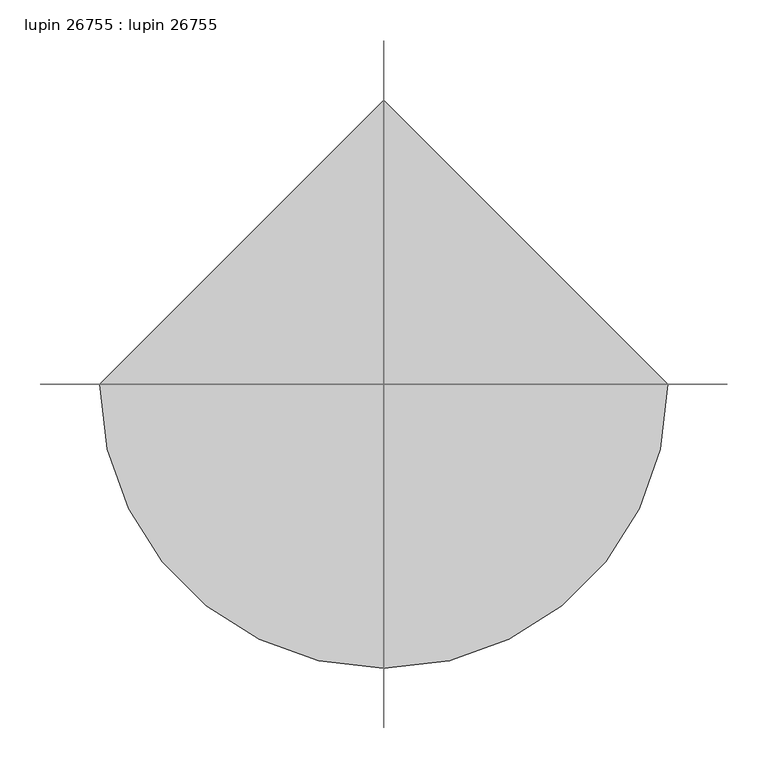
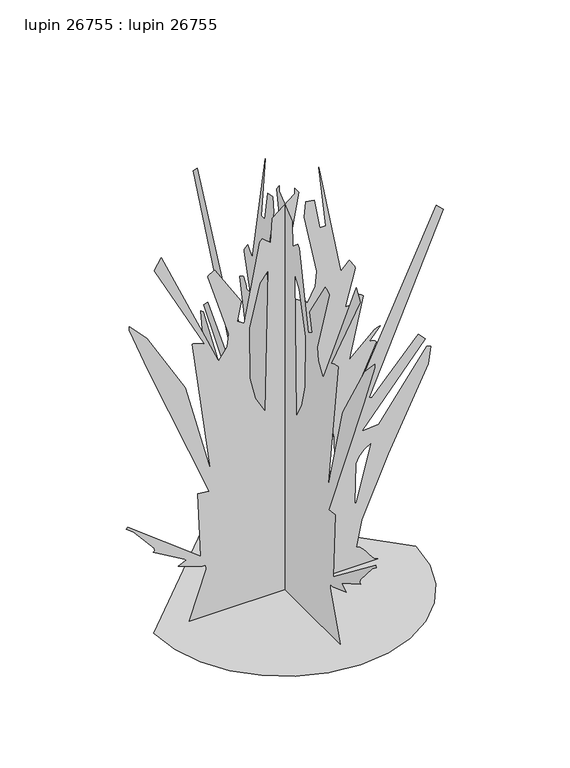
"""IFC4 building model written with IfcOpenShell, lengths in millimetres: proxy geometry, lupin 26755 : lupin 26755."""

import ifcopenshell
import ifcopenshell.guid

model = None  # the IFC model being written
_history = None  # IfcOwnerHistory: only IFC2X3 demands one
_inside = {}  # id of a spatial element -> (the spatial element, [elements in it])
_under = {}  # id of a project, library or spatial element -> (it, [spatial elements below it])
_declared = {}  # id of a project -> (the project, [libraries it declares])
_typed = {}  # id of a type object -> (the type object, [elements of that type])
_made_of = {}  # id of a material, layer set ... -> (it, [elements and type objects made of it])


def new_model(schema):
    """Start an empty IFC model of exactly this schema.

    Asked for "IFC4X3", IfcOpenShell would pick the latest addendum, in which some entities
    have other attributes; the version numbers below select the first issue.
    IFC2X3 requires an IfcOwnerHistory on every rooted entity: one is made here for all.
    """
    global model, _history
    if schema == "IFC4X3":
        model = ifcopenshell.file(schema_version=(4, 3, 0, 0))
    else:
        model = ifcopenshell.file(schema=schema)
    _inside.clear()
    _under.clear()
    _declared.clear()
    _typed.clear()
    _made_of.clear()
    _history = None
    if model.schema == "IFC2X3":
        org = make("IfcOrganization", Name="unknown")
        user = make(
            "IfcPersonAndOrganization",
            ThePerson=make("IfcPerson", FamilyName="unknown"),
            TheOrganization=org,
        )
        app = make(
            "IfcApplication",
            ApplicationDeveloper=org,
            Version="unknown",
            ApplicationFullName="unknown",
            ApplicationIdentifier="unknown",
        )
        _history = make(
            "IfcOwnerHistory",
            OwningUser=user,
            OwningApplication=app,
            ChangeAction="ADDED",
            CreationDate=0,
        )
    return model


def make(cls, **values):
    """One entity of the class cls with the attributes given. An attribute that is None is left unset."""
    return model.create_entity(
        cls, **{name: value for name, value in values.items() if value is not None}
    )


def rooted(cls, **values):
    """An entity with a GlobalId (a new one), such as an element, a storey or a relation."""
    return make(cls, GlobalId=ifcopenshell.guid.new(), OwnerHistory=_history, **values)


def si_unit(unit_type, name, prefix=None):
    """IfcSIUnit, for example si_unit("LENGTHUNIT", "METRE", prefix="MILLI")."""
    return make("IfcSIUnit", UnitType=unit_type, Prefix=prefix, Name=name)


def assignment(units):
    """IfcUnitAssignment: the units of a project."""
    return None if units is None else make("IfcUnitAssignment", Units=units)


def point(xyz):
    """IfcCartesianPoint."""
    return None if xyz is None else make("IfcCartesianPoint", Coordinates=xyz)


def direction(xyz):
    """IfcDirection."""
    return None if xyz is None else make("IfcDirection", DirectionRatios=xyz)


def frame(location, z_axis=None, x_axis=None):
    """IfcAxis2Placement3D, a coordinate frame: its origin and axes. An axis left out is left unset."""
    return make(
        "IfcAxis2Placement3D",
        Location=point(location),
        Axis=direction(z_axis),
        RefDirection=direction(x_axis),
    )


def origin():
    """The frame at (0, 0, 0) with its axes left unset."""
    return frame((0.0, 0.0, 0.0))


def place(relative_to, where):
    """IfcLocalPlacement: puts the frame where relative to a parent placement (None: the world)."""
    return make(
        "IfcLocalPlacement", PlacementRelTo=relative_to, RelativePlacement=where
    )


def context(
    kind, dimensions, precision=None, world=None, true_north=None, identifier=None
):
    """IfcGeometricRepresentationContext, for example the 3D "Model" context."""
    return make(
        "IfcGeometricRepresentationContext",
        ContextIdentifier=identifier,
        ContextType=kind,
        CoordinateSpaceDimension=dimensions,
        Precision=precision,
        WorldCoordinateSystem=world,
        TrueNorth=true_north,
    )


def project(units=None, contexts=None):
    """IfcProject with its units and contexts."""
    return rooted(
        "IfcProject",
        Name="project",
        RepresentationContexts=contexts,
        UnitsInContext=assignment(units),
    )


def spatial(cls, under=None, at=None, **own):
    """A site, building, storey or space (cls), placed at a placement, below another one or the project."""
    s = rooted(cls, ObjectPlacement=at, **own)
    if under is not None:
        _under.setdefault(under.id(), (under, []))[1].append(s)
    return s


def point_list(points):
    """IfcCartesianPointList2D or 3D."""
    cls = (
        "IfcCartesianPointList2D" if len(points[0]) == 2 else "IfcCartesianPointList3D"
    )
    return make(cls, CoordList=points)


def triangles(points, corners, closed=None, point_numbers=None):
    """IfcTriangulatedFaceSet: each triangle names its three corners, points numbered from 1."""
    return make(
        "IfcTriangulatedFaceSet",
        Coordinates=point_list(points),
        Closed=closed,
        CoordIndex=corners,
        PnIndex=point_numbers,
    )


def shape(context_of_items, identifier, shape_type, items):
    """IfcShapeRepresentation: the items that make up one representation, for example the "Body"."""
    return make(
        "IfcShapeRepresentation",
        ContextOfItems=context_of_items,
        RepresentationIdentifier=identifier,
        RepresentationType=shape_type,
        Items=items,
    )


def source(mapping_origin, context_of_items, identifier, shape_type, items):
    """IfcRepresentationMap: a shape defined once, which mapped items show again and again."""
    return make(
        "IfcRepresentationMap",
        MappingOrigin=mapping_origin,
        MappedRepresentation=shape(context_of_items, identifier, shape_type, items),
    )


def transform(
    local_origin,
    x_axis=None,
    y_axis=None,
    z_axis=None,
    scale=None,
    scale2=None,
    scale3=None,
    uniform=True,
):
    """IfcCartesianTransformationOperator3D, or its non-uniform kind. x_axis, y_axis, z_axis: its Axis1, 2, 3."""
    if uniform:
        return make(
            "IfcCartesianTransformationOperator3D",
            Axis1=direction(x_axis),
            Axis2=direction(y_axis),
            LocalOrigin=point(local_origin),
            Scale=scale,
            Axis3=direction(z_axis),
        )
    return make(
        "IfcCartesianTransformationOperator3DnonUniform",
        Axis1=direction(x_axis),
        Axis2=direction(y_axis),
        LocalOrigin=point(local_origin),
        Scale=scale,
        Axis3=direction(z_axis),
        Scale2=scale2,
        Scale3=scale3,
    )


def mapped(mapping_source, mapping_target):
    """IfcMappedItem: shows the shape of a source again, moved by a transform."""
    return make(
        "IfcMappedItem", MappingSource=mapping_source, MappingTarget=mapping_target
    )


def made_of(thing, what):
    """Note that an element or type object is made of a material, layer set ...; save() writes the relation."""
    if what is not None:
        _made_of.setdefault(what.id(), (what, []))[1].append(thing)
    return thing


def element(
    cls,
    number,
    at=None,
    inside=None,
    cuts=None,
    type_object=None,
    material=None,
    context=None,
    identifier="Body",
    shape_type=None,
    held_by="IfcProductDefinitionShape",
    body=None,
    shapes=None,
    **own,
):
    """One element of the class cls, such as IfcWall. Its Tag is "e" and its number.

    at: its placement. inside: the storey or other place that contains it. cuts: it is an
    opening in that element (IfcRelVoidsElement). A single representation is given by context,
    identifier, shape_type and body (its items); several are given by shapes. held_by: the class
    of the entity that holds the representations. save() writes the other relations.
    """
    e = rooted(cls, Tag="e%d" % number, ObjectPlacement=at, **own)
    if body is not None:
        shapes = [shape(context, identifier, shape_type, body)]
    if shapes is not None:
        e.Representation = make(held_by, Representations=shapes)
    if inside is not None:
        _inside.setdefault(inside.id(), (inside, []))[1].append(e)
    if cuts is not None:
        rooted(
            "IfcRelVoidsElement", RelatingBuildingElement=cuts, RelatedOpeningElement=e
        )
    if type_object is not None:
        _typed.setdefault(type_object.id(), (type_object, []))[1].append(e)
    return made_of(e, material)


def aggregate(whole, parts):
    """IfcRelAggregates: a whole, such as a stair, and the parts it consists of."""
    return rooted("IfcRelAggregates", RelatingObject=whole, RelatedObjects=parts)


def save(model, path):
    """Write the relations noted so far, then the file.

    IfcRelAggregates (storeys below a building ...), IfcRelContainedInSpatialStructure (elements
    in a storey), IfcRelDefinesByType, IfcRelAssociatesMaterial and IfcRelDeclares: one each for
    every whole, place, type object, material and project.
    """
    for whole, parts in _under.values():
        aggregate(whole, parts)
    for where, things in _inside.values():
        rooted(
            "IfcRelContainedInSpatialStructure",
            RelatedElements=things,
            RelatingStructure=where,
        )
    for kind, things in _typed.values():
        rooted("IfcRelDefinesByType", RelatedObjects=things, RelatingType=kind)
    for what, things in _made_of.values():
        rooted("IfcRelAssociatesMaterial", RelatedObjects=things, RelatingMaterial=what)
    for by, libraries in _declared.values():
        rooted("IfcRelDeclares", RelatingContext=by, RelatedDefinitions=libraries)
    model.write(path)


def lupin_26755_lupin_26755_1db73bb0(model_context):
    return source(origin(), model_context, "Body", "Tessellation", [
        triangles([(-351.9469769, 0.0, 0.0), (-342.6429663, -80.6431063, 0.0), (-316.1457464, -154.7010223, 0.0), (-274.573611, -220.0515756, 0.0), (-220.0515756, -274.573611, 0.0), (-154.700768, -316.1457464, 0.0), (-80.6431063, -342.6429663, 0.0), (1.54e-05, -351.9469769, 0.0), (80.6431063, -342.6429663, 0.0), (154.7010223, -316.1457464, 0.0), (220.0515756, -274.573611, 0.0), (274.573611, -220.0515756, 0.0), (316.1457464, -154.700768, 0.0), (342.6429663, -80.6431063, 0.0), (351.9469769, 3.08e-05, 0.0), (-4.62e-05, 351.9469769, 0.0), (150.6720804, -0.0015947, 851.9910187), (173.2724542, -0.0015961, 874.5918921), (188.3394669, -0.0015947, 851.9910187), (188.5203062, -0.0015944, 847.0684994), (161.9722718, -0.0015884, 746.5202036), (177.0392664, -0.0015884, 746.5202036), (178.9694175, -0.0015886, 750.284436), (180.6039107, -0.0015889, 754.0461977), (182.1639718, -0.0015891, 757.8054159), (183.8723704, -0.0015893, 761.5671049), (185.9508409, -0.0015895, 765.3339535), (188.6214083, -0.0015898, 769.1058163), (192.1062791, -0.00159, 772.8878529), (193.2812801, -0.00159, 772.4611347), (195.5106317, -0.0015899, 771.3080074), (198.4649026, -0.0015898, 769.6264967), (201.8143893, -0.0015897, 767.6173897), (205.2296787, -0.0015896, 765.4761686), (208.3815575, -0.0015894, 763.4010046), (210.9401041, -0.0015893, 761.5874525), (173.2724542, -0.0015792, 592.0833366), (240.700733, -0.0015829, 654.2395718), (250.6943454, -0.0015832, 659.6218014), (256.1408516, -0.0015833, 659.8859568), (226.0070987, -0.0015812, 625.984683), (228.5658996, -0.0015812, 626.1598904), (231.7175241, -0.0015812, 625.7001801), (235.1327953, -0.0015812, 624.7324339), (238.4825545, -0.0015811, 623.3938528), (241.4365711, -0.001581, 621.8114639), (243.6659227, -0.0015809, 620.1197794), (244.8409236, -0.0015808, 618.4509859), (180.8060786, -0.0015725, 479.0814042), (184.572909, -0.0015725, 479.0814042), (406.8108882, -0.0016005, 949.9256659), (425.6449857, -0.0015994, 931.0915684), (226.0070987, -0.0015718, 467.7809675), (233.5407231, -0.0015716, 464.0141553), (357.8448363, -0.0015797, 599.6169611), (376.6763904, -0.0015785, 580.7828636), (207.1732737, -0.0015664, 377.3799811), (252.3745481, -0.0015666, 381.1467934), (380.4432026, -0.0015772, 558.1819902), (391.7436393, -0.001577, 554.4177215), (384.6443633, -0.0015741, 506.8385036), (278.1600926, -0.0015612, 289.3386073), (206.7572381, -0.0015515, 126.6752076), (192.1062791, -0.0015471, 53.437713), (201.6487926, -0.0015469, 49.4892894), (210.1163717, -0.0015464, 41.8553304), (217.9390592, -0.0015458, 32.010051), (225.5471159, -0.0015452, 21.427562), (233.3697852, -0.0015446, 11.5823576), (241.8373824, -0.0015442, 3.9483989), (251.3798959, -0.0015439, 1.66e-05), (-256.5091613, -0.001544, 0.4898205), (-211.4973739, -0.0015518, 132.0554297), (-212.2487088, -0.0015525, 144.4635658), (-222.2372343, -0.0015525, 143.8397394), (-286.2728424, -0.0015538, 166.4403676), (-263.6719508, -0.0015545, 177.7405681), (-354.0729735, -0.0015577, 230.4752126), (-348.9472326, -0.0015578, 232.5839138), (-351.022433, -0.0015583, 241.0403199), (-406.3257797, -0.0015621, 305.3939318), (-425.6424422, -0.0015631, 320.8777614), (-421.87563, -0.0015633, 324.6445736), (-226.0037922, -0.0015543, 173.9740102), (-233.5374348, -0.0015651, 354.7790714), (-203.4034275, -0.0015648, 351.0122592), (-366.5443417, -0.0015886, 750.3606668), (-417.7760619, -0.0015966, 882.9891266), (-418.1088178, -0.0015972, 893.4259169), (-370.8775801, -0.0015942, 843.3371864), (-268.1575782, -0.0015837, 667.2316566), (-199.6365971, -0.0015682, 407.5119355), (-248.6044294, -0.0015907, 784.1883259), (-246.3971695, -0.0015907, 784.2213181), (-242.3227634, -0.0015906, 783.3755121), (-236.9745433, -0.0015905, 781.8490065), (-230.9453692, -0.0015904, 779.8398268), (-224.8285369, -0.0015903, 777.5436733), (-219.2169245, -0.0015901, 775.1611879), (-214.7036098, -0.00159, 772.8878529), (-350.306125, -0.0016053, 1029.028759), (-331.4720638, -0.0016071, 1059.1632568), (-180.8027903, -0.0015866, 716.3881765), (-177.0359781, -0.0015864, 712.6214006), (-155.1577168, -0.0015883, 744.8692142), (-150.1099781, -0.0015904, 779.1769312), (-207.1702397, -0.0016012, 961.2260662), (-205.9949844, -0.0016013, 963.0370749), (-203.7656147, -0.0016014, 965.1147823), (-194.0468402, -0.0016018, 970.9440777), (-190.8949614, -0.0016019, 972.0972776), (-188.3364148, -0.0016019, 972.5265392), (-116.7679544, -0.0015952, 859.5246431), (-128.0681458, -0.001592, 806.7891993), (-109.2343208, -0.0015913, 795.4887989), (-67.8001221, -0.0016041, 1010.1946615), (-60.2664931, -0.0016046, 1017.728286), (-37.6658604, -0.0016035, 998.8941885), (-33.8993003, -0.0016075, 1066.6968813), (26.3689732, -0.0016104, 1115.6629332), (26.3689732, -0.0016113, 1130.7301821), (37.6691624, -0.0016104, 1115.6629332), (2.9836067, -0.0015988, 921.19319), (5.2254839, -0.0015953, 862.2830503), (21.4607608, -0.0015927, 818.4376162), (56.5029828, -0.0015916, 799.2555748), (60.269795, -0.0015911, 791.7219503), (81.2288264, -0.0015936, 833.4109028), (86.0914021, -0.0015961, 874.8052511), (51.7460784, -0.0016059, 1039.955781), (56.5029828, -0.0016084, 1081.7615868), (79.10362, -0.0016082, 1077.9948109), (94.1706237, -0.0016032, 995.1274126), (109.237373, -0.0016032, 995.1274126), (90.4038023, -0.0016136, 1168.3983044), (-67.325905, -0.0015972, 893.4183592), (-96.1172708, -0.0015902, 776.6851501), (-94.9783414, -0.0015817, 633.9373953), (-79.6923831, -0.001578, 571.2782112), (-52.7331184, -0.0015752, 524.2831873), (-45.1994894, -0.001599, 923.5579439), (109.237373, -0.0015608, 283.2096027), (135.6048224, -0.0015619, 302.0436639), (131.8382554, -0.0015682, 407.5119355), (211.912919, -0.0015632, 322.7039944), (198.2078507, -0.0015623, 307.9059877), (189.9752137, -0.0015612, 290.5146256), (188.3394669, -0.0015547, 181.5073803), (192.1062791, -0.0015545, 177.7405681), (232.2618404, -0.0015639, 335.5792259), (0.0016106, 150.6687739, 851.9910187), (0.0016109, 173.269402, 874.5918921), (0.00161, 188.3364148, 851.9910187), (0.0016099, 188.5169997, 847.0684994), (0.0016073, 161.9689653, 746.5202036), (0.001607, 177.0362324, 746.5202036), (0.0016071, 178.9663653, 750.284436), (0.0016072, 180.6006042, 754.0461977), (0.0016073, 182.1609196, 757.8054159), (0.0016074, 183.8693182, 761.5671049), (0.0016075, 185.9478069, 765.3339535), (0.0016076, 188.6183561, 769.1058163), (0.0016076, 192.103227, 772.8878529), (0.0016076, 193.2782279, 772.4611347), (0.0016075, 195.5075795, 771.3080074), (0.0016074, 198.4615962, 769.6264967), (0.0016073, 201.8113554, 767.6173897), (0.0016072, 205.2266265, 765.4761686), (0.0016071, 208.378251, 763.4010046), (0.001607, 210.937052, 761.5874525), (0.0016025, 173.269402, 592.0833366), (0.0016033, 240.6974266, 654.2395718), (0.0016034, 250.6910389, 659.6218014), (0.0016033, 256.1383082, 659.8859568), (0.0016027, 226.0040465, 625.984683), (0.0016027, 228.5625931, 626.1598904), (0.0016026, 231.7142176, 625.7001801), (0.0016026, 235.1297431, 624.7324339), (0.0016025, 238.479248, 623.3938528), (0.0016024, 241.4332646, 621.8114639), (0.0016023, 243.6626162, 620.1197794), (0.0016022, 244.8378715, 618.4509859), (0.001599, 180.8027903, 479.0814042), (0.001599, 184.5696025, 479.0814042), (0.0016097, 406.8083447, 949.9256659), (0.0016088, 425.6424422, 931.0915684), (0.001598, 226.0040465, 467.7809675), (0.0015978, 233.5374348, 464.0141553), (0.0016, 357.8397858, 599.6169611), (0.0015991, 376.6738469, 580.7828636), (0.0015956, 207.1702397, 377.3799811), (0.001595, 252.3712416, 381.1467934), (0.0015984, 380.4406591, 558.1845337), (0.0015981, 391.7410958, 554.4177215), (0.0015968, 384.6418199, 506.8385036), (0.0015919, 278.1575492, 289.3386073), (0.0015881, 206.7539316, 126.6752076), (0.0015862, 192.103227, 53.437713), (0.0015859, 201.6454861, 49.4892894), (0.0015856, 210.1130652, 41.8553304), (0.0015851, 217.936007, 32.010051), (0.0015847, 225.5438094, 21.427587), (0.0015843, 233.3664787, 11.5823837), (0.001584, 241.8343303, 3.9483989), (0.0015837, 251.3765894, 2.41e-05), (0.0015913, -256.51423, 0.4898434), (0.0015945, -211.5006804, 132.0554297), (0.0015949, -212.2519971, 144.4635658), (0.001595, -222.2402864, 143.8397394), (0.0015967, -286.2753676, 166.4403676), (0.0015967, -263.6744943, 177.7405681), (0.0015996, -354.0780241, 230.4752126), (0.0015996, -348.9497761, 232.5839138), (0.0015999, -351.0249764, 241.0403199), (0.0016026, -406.3308303, 305.3939318), (0.0016033, -425.6449857, 320.8777614), (0.0016034, -421.8781734, 324.6445736), (0.001596, -226.0070987, 173.9740102), (0.0016015, -233.5404688, 354.7790714), (0.0016009, -203.4064615, 351.0122592), (0.0016153, -366.5468851, 750.3606668), (0.00162, -417.7786054, 882.9891266), (0.0016203, -418.1113612, 893.4259169), (0.0016181, -370.8801235, 843.3371864), (0.0016113, -268.1626651, 667.2316566), (0.0016026, -199.6396492, 407.5119355), (0.0016145, -248.6077359, 784.1883259), (0.0016145, -246.4002216, 784.2213181), (0.0016144, -242.3260699, 783.3755121), (0.0016143, -236.9775955, 781.8490065), (0.0016141, -230.9484032, 779.8398268), (0.001614, -224.8318434, 777.5436733), (0.0016138, -219.2199766, 775.1611879), (0.0016137, -214.7069163, 772.8878529), (0.0016233, -350.3112119, 1029.028759), (0.0016239, -331.4771507, 1059.1632568), (0.0016115, -180.8060786, 716.3881765), (0.0016113, -177.0392664, 712.6214006), (0.001612, -155.1607508, 744.8692142), (0.0016129, -150.1132755, 779.1769312), (0.0016192, -207.1732737, 961.2260662), (0.0016192, -205.9982728, 963.0396183), (0.0016192, -203.7689212, 965.1147823), (0.0016193, -194.0498742, 970.9466211), (0.0016193, -190.8979953, 972.0998211), (0.0016192, -188.3394669, 972.5265392), (0.0016148, -116.7709974, 859.5246431), (0.0016134, -128.0714432, 806.7891993), (0.0016128, -109.2376273, 795.4887989), (0.0016186, -67.8031697, 1010.1946615), (0.0016187, -60.269795, 1017.728286), (0.0016178, -37.6691624, 998.8941885), (0.0016197, -33.9023479, 1066.6968813), (0.0016203, 26.3656713, 1115.6629332), (0.0016207, 26.3656713, 1130.7301821), (0.0016201, 37.6661148, 1115.6629332), (0.0016148, 2.9804319, 921.19319), (0.0016131, 5.2223085, 862.2830503), (0.0016115, 21.4575588, 818.4376162), (0.0016104, 56.4999352, 799.2555748), (0.0016101, 60.2664931, 791.7219503), (0.0016111, 81.225529, 833.4109028), (0.0016122, 86.0883499, 874.8052511), (0.0016177, 51.7430263, 1039.955781), (0.0016188, 56.4999352, 1081.7615868), (0.0016184, 79.1003135, 1077.9948109), (0.0016157, 94.1673172, 995.1274126), (0.0016155, 109.2340665, 995.1274126), (0.0016209, 90.4007593, 1168.3983044), (0.0016151, -67.329207, 893.4183592), (0.001612, -96.120323, 776.6851501), (0.0016077, -94.9816388, 633.9373953), (0.0016057, -79.6956896, 571.2782112), (0.0016039, -52.736166, 524.2831873), (0.0016156, -45.202537, 923.5579439), (0.0015943, 109.2340665, 283.2096027), (0.0015944, 135.6017703, 302.0436639), (0.0015976, 131.834958, 407.5119355), (0.0015939, 211.9098669, 322.7039944), (0.0015937, 198.2045624, 307.9059877), (0.0015933, 189.9719254, 290.5146256), (0.00159, 188.3364148, 181.5073803), (0.0015899, 192.103227, 177.7405681), (0.001594, 232.2587883, 335.5792259)], [[15, 16, 1], [14, 15, 1], [14, 1, 2], [13, 14, 2], [13, 2, 3], [13, 3, 4], [12, 13, 4], [11, 12, 4], [11, 4, 5], [11, 5, 6], [11, 6, 7], [11, 7, 8], [11, 8, 9], [11, 9, 10], [144, 142, 18], [134, 135, 17], [70, 71, 72], [120, 121, 122], [17, 18, 142], [140, 17, 142], [88, 89, 90], [69, 70, 72], [39, 40, 41], [38, 39, 41], [37, 38, 41], [75, 76, 77], [77, 78, 79], [68, 69, 72], [101, 102, 103], [100, 101, 103], [67, 68, 72], [66, 67, 72], [65, 66, 72], [64, 65, 72], [147, 148, 143], [50, 51, 52], [50, 52, 53], [119, 120, 122], [118, 119, 122], [142, 143, 148], [84, 85, 86], [64, 72, 73], [92, 93, 94], [92, 94, 95], [92, 95, 96], [92, 96, 97], [92, 97, 98], [92, 98, 99], [92, 99, 100], [92, 100, 103], [92, 103, 104], [81, 82, 83], [81, 83, 84], [80, 81, 84], [79, 80, 84], [77, 79, 84], [75, 77, 84], [130, 131, 132], [130, 132, 133], [54, 55, 56], [54, 56, 57], [63, 64, 73], [87, 88, 90], [87, 90, 91], [87, 91, 92], [86, 87, 92], [74, 75, 84], [63, 73, 74], [116, 117, 118], [115, 116, 118], [118, 122, 123], [53, 54, 57], [50, 53, 57], [59, 60, 61], [58, 59, 61], [58, 61, 62], [57, 58, 62], [49, 50, 57], [146, 147, 143], [146, 143, 144], [145, 146, 144], [150, 145, 144], [133, 134, 17], [130, 133, 17], [129, 130, 17], [128, 129, 17], [128, 17, 140], [127, 128, 140], [28, 29, 30], [35, 36, 37], [34, 35, 37], [33, 34, 37], [32, 33, 37], [31, 32, 37], [30, 31, 37], [28, 30, 37], [27, 28, 37], [26, 27, 37], [25, 26, 37], [24, 25, 37], [23, 24, 37], [22, 23, 37], [21, 22, 37], [111, 112, 113], [110, 111, 113], [109, 110, 113], [108, 109, 113], [107, 108, 113], [107, 113, 114], [106, 107, 114], [63, 74, 84], [63, 84, 86], [63, 86, 92], [47, 48, 49], [46, 47, 49], [45, 46, 49], [44, 45, 49], [43, 44, 49], [42, 43, 49], [41, 42, 49], [37, 41, 49], [63, 92, 104], [105, 106, 114], [105, 114, 115], [126, 127, 140], [125, 126, 140], [125, 140, 141], [124, 125, 141], [123, 124, 141], [118, 123, 141], [118, 141, 136], [115, 118, 136], [115, 136, 137], [105, 115, 137], [104, 105, 137], [104, 137, 138], [104, 138, 139], [18, 19, 20], [18, 20, 21], [144, 18, 21], [144, 21, 37], [144, 37, 49], [144, 49, 57], [150, 144, 57], [150, 57, 62], [149, 150, 62], [149, 62, 63], [148, 149, 63], [142, 148, 63], [104, 139, 140], [63, 104, 140], [63, 140, 142], [278, 276, 152], [268, 269, 151], [204, 205, 206], [254, 255, 256], [151, 152, 276], [274, 151, 276], [222, 223, 224], [203, 204, 206], [173, 174, 175], [172, 173, 175], [171, 172, 175], [209, 210, 211], [211, 212, 213], [202, 203, 206], [235, 236, 237], [234, 235, 237], [201, 202, 206], [200, 201, 206], [199, 200, 206], [198, 199, 206], [281, 282, 277], [184, 185, 186], [184, 186, 187], [253, 254, 256], [252, 253, 256], [276, 277, 282], [218, 219, 220], [198, 206, 207], [226, 227, 228], [226, 228, 229], [226, 229, 230], [226, 230, 231], [226, 231, 232], [226, 232, 233], [226, 233, 234], [226, 234, 237], [226, 237, 238], [215, 216, 217], [215, 217, 218], [214, 215, 218], [213, 214, 218], [211, 213, 218], [209, 211, 218], [264, 265, 266], [264, 266, 267], [188, 189, 190], [188, 190, 191], [197, 198, 207], [221, 222, 224], [221, 224, 225], [221, 225, 226], [220, 221, 226], [208, 209, 218], [197, 207, 208], [250, 251, 252], [249, 250, 252], [252, 256, 257], [187, 188, 191], [184, 187, 191], [193, 194, 195], [192, 193, 195], [192, 195, 196], [191, 192, 196], [183, 184, 191], [280, 281, 277], [280, 277, 278], [279, 280, 278], [284, 279, 278], [267, 268, 151], [264, 267, 151], [263, 264, 151], [262, 263, 151], [262, 151, 274], [261, 262, 274], [162, 163, 164], [169, 170, 171], [168, 169, 171], [167, 168, 171], [166, 167, 171], [165, 166, 171], [164, 165, 171], [162, 164, 171], [161, 162, 171], [160, 161, 171], [159, 160, 171], [158, 159, 171], [157, 158, 171], [156, 157, 171], [155, 156, 171], [245, 246, 247], [244, 245, 247], [243, 244, 247], [242, 243, 247], [241, 242, 247], [241, 247, 248], [240, 241, 248], [197, 208, 218], [197, 218, 220], [197, 220, 226], [181, 182, 183], [180, 181, 183], [179, 180, 183], [178, 179, 183], [177, 178, 183], [176, 177, 183], [175, 176, 183], [171, 175, 183], [197, 226, 238], [239, 240, 248], [239, 248, 249], [260, 261, 274], [259, 260, 274], [259, 274, 275], [258, 259, 275], [257, 258, 275], [252, 257, 275], [252, 275, 270], [249, 252, 270], [249, 270, 271], [239, 249, 271], [238, 239, 271], [238, 271, 272], [238, 272, 273], [152, 153, 154], [152, 154, 155], [278, 152, 155], [278, 155, 171], [278, 171, 183], [278, 183, 191], [284, 278, 191], [284, 191, 196], [283, 284, 196], [283, 196, 197], [282, 283, 197], [276, 282, 197], [238, 273, 274], [197, 238, 274], [197, 274, 276]], closed=False),
    ])


if __name__ == "__main__":
    model = new_model("IFC4")
    model_context = context("Model", 3, world=origin())
    ifc_project = project(units=[si_unit("LENGTHUNIT", "METRE", prefix="MILLI")], contexts=[model_context])
    site = spatial("IfcSite", under=ifc_project)
    building = spatial("IfcBuilding", under=site)
    placement = place(None, origin())
    lupin_26755_lupin_26755_shape = lupin_26755_lupin_26755_1db73bb0(model_context)
    element("IfcBuildingElementProxy", 1, Name="lupin 26755 : lupin 26755", ObjectType="lupin 26755 : lupin 26755", at=placement, inside=building, context=model_context, shape_type="MappedRepresentation", body=[
        mapped(lupin_26755_lupin_26755_shape, transform((0.0, 0.0, 0.0), x_axis=(1.0, 0.0, 0.0), y_axis=(0.0, 1.0, 0.0), z_axis=(0.0, 0.0, 1.0))),
    ])
    save(model, "model.ifc")

# Revit data of these elements
# Project information
#   Project Issue Date = "Issue Date"
#   Project Status = "Project Status"
#   Client Name = "Owner"
#   Project Address = "Enter address here"
#   Project Name = "Project Name"
#   Project Number = "Project Number"
# Type "lupin 26755 : lupin 26755"
#   built-in parameter 1005195 = "RPC-16-G2M4-C67X-C72M-U000-ST1L-LVER-AU"
#   Height = 0
